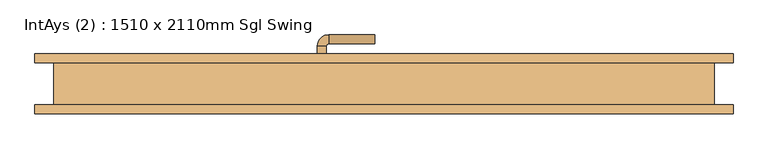
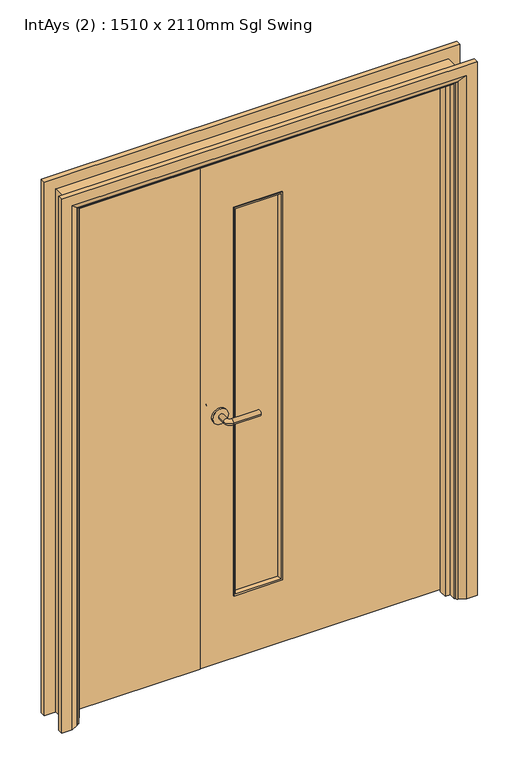
"""IFC4 building model written with IfcOpenShell, lengths in millimetres: door geometry, IntAys (2) : 1510 x 2110mm Sgl Swing."""

import ifcopenshell
import ifcopenshell.guid

model = None  # the IFC model being written
_history = None  # IfcOwnerHistory: only IFC2X3 demands one
_inside = {}  # id of a spatial element -> (the spatial element, [elements in it])
_under = {}  # id of a project, library or spatial element -> (it, [spatial elements below it])
_declared = {}  # id of a project -> (the project, [libraries it declares])
_typed = {}  # id of a type object -> (the type object, [elements of that type])
_made_of = {}  # id of a material, layer set ... -> (it, [elements and type objects made of it])


def new_model(schema):
    """Start an empty IFC model of exactly this schema.

    Asked for "IFC4X3", IfcOpenShell would pick the latest addendum, in which some entities
    have other attributes; the version numbers below select the first issue.
    IFC2X3 requires an IfcOwnerHistory on every rooted entity: one is made here for all.
    """
    global model, _history
    if schema == "IFC4X3":
        model = ifcopenshell.file(schema_version=(4, 3, 0, 0))
    else:
        model = ifcopenshell.file(schema=schema)
    _inside.clear()
    _under.clear()
    _declared.clear()
    _typed.clear()
    _made_of.clear()
    _history = None
    if model.schema == "IFC2X3":
        org = make("IfcOrganization", Name="unknown")
        user = make(
            "IfcPersonAndOrganization",
            ThePerson=make("IfcPerson", FamilyName="unknown"),
            TheOrganization=org,
        )
        app = make(
            "IfcApplication",
            ApplicationDeveloper=org,
            Version="unknown",
            ApplicationFullName="unknown",
            ApplicationIdentifier="unknown",
        )
        _history = make(
            "IfcOwnerHistory",
            OwningUser=user,
            OwningApplication=app,
            ChangeAction="ADDED",
            CreationDate=0,
        )
    return model


def make(cls, **values):
    """One entity of the class cls with the attributes given. An attribute that is None is left unset."""
    return model.create_entity(
        cls, **{name: value for name, value in values.items() if value is not None}
    )


def rooted(cls, **values):
    """An entity with a GlobalId (a new one), such as an element, a storey or a relation."""
    return make(cls, GlobalId=ifcopenshell.guid.new(), OwnerHistory=_history, **values)


def si_unit(unit_type, name, prefix=None):
    """IfcSIUnit, for example si_unit("LENGTHUNIT", "METRE", prefix="MILLI")."""
    return make("IfcSIUnit", UnitType=unit_type, Prefix=prefix, Name=name)


def assignment(units):
    """IfcUnitAssignment: the units of a project."""
    return None if units is None else make("IfcUnitAssignment", Units=units)


def point(xyz):
    """IfcCartesianPoint."""
    return None if xyz is None else make("IfcCartesianPoint", Coordinates=xyz)


def direction(xyz):
    """IfcDirection."""
    return None if xyz is None else make("IfcDirection", DirectionRatios=xyz)


def frame(location, z_axis=None, x_axis=None):
    """IfcAxis2Placement3D, a coordinate frame: its origin and axes. An axis left out is left unset."""
    return make(
        "IfcAxis2Placement3D",
        Location=point(location),
        Axis=direction(z_axis),
        RefDirection=direction(x_axis),
    )


def frame_2d(location, x_axis=None):
    """IfcAxis2Placement2D, a coordinate frame in the plane: its origin and x axis."""
    return make(
        "IfcAxis2Placement2D", Location=point(location), RefDirection=direction(x_axis)
    )


def origin():
    """The frame at (0, 0, 0) with its axes left unset."""
    return frame((0.0, 0.0, 0.0))


def place(relative_to, where):
    """IfcLocalPlacement: puts the frame where relative to a parent placement (None: the world)."""
    return make(
        "IfcLocalPlacement", PlacementRelTo=relative_to, RelativePlacement=where
    )


def context(
    kind, dimensions, precision=None, world=None, true_north=None, identifier=None
):
    """IfcGeometricRepresentationContext, for example the 3D "Model" context."""
    return make(
        "IfcGeometricRepresentationContext",
        ContextIdentifier=identifier,
        ContextType=kind,
        CoordinateSpaceDimension=dimensions,
        Precision=precision,
        WorldCoordinateSystem=world,
        TrueNorth=true_north,
    )


def project(units=None, contexts=None):
    """IfcProject with its units and contexts."""
    return rooted(
        "IfcProject",
        Name="project",
        RepresentationContexts=contexts,
        UnitsInContext=assignment(units),
    )


def spatial(cls, under=None, at=None, **own):
    """A site, building, storey or space (cls), placed at a placement, below another one or the project."""
    s = rooted(cls, ObjectPlacement=at, **own)
    if under is not None:
        _under.setdefault(under.id(), (under, []))[1].append(s)
    return s


def polyline(points):
    """IfcPolyline through the points."""
    return make("IfcPolyline", Points=[point(p) for p in points])


def circle_curve(where, radius):
    """IfcCircle in the frame where."""
    return make("IfcCircle", Position=where, Radius=radius)


def ellipse_curve(where, semi_axis1, semi_axis2):
    """IfcEllipse in the frame where."""
    return make(
        "IfcEllipse", Position=where, SemiAxis1=semi_axis1, SemiAxis2=semi_axis2
    )


def trimmed(basis, trim1, trim2, sense, master):
    """IfcTrimmedCurve: the piece of a basis curve between two trims."""
    return make(
        "IfcTrimmedCurve",
        BasisCurve=basis,
        Trim1=trim1,
        Trim2=trim2,
        SenseAgreement=sense,
        MasterRepresentation=master,
    )


def segment(curve, same_sense, transition):
    """IfcCompositeCurveSegment."""
    return make(
        "IfcCompositeCurveSegment",
        Transition=transition,
        SameSense=same_sense,
        ParentCurve=curve,
    )


def composite_curve(segments, self_intersect=None):
    """IfcCompositeCurve: segments joined end to end."""
    return make("IfcCompositeCurve", Segments=segments, SelfIntersect=self_intersect)


def outline(outer, holes=None, kind="AREA"):
    """IfcArbitraryClosedProfileDef: a profile drawn as a closed curve; with holes, ...WithVoids."""
    if holes is None:
        return make("IfcArbitraryClosedProfileDef", ProfileType=kind, OuterCurve=outer)
    return make(
        "IfcArbitraryProfileDefWithVoids",
        ProfileType=kind,
        OuterCurve=outer,
        InnerCurves=holes,
    )


def extrude(swept, where, along, depth):
    """IfcExtrudedAreaSolid: the profile swept, set in the frame where, extruded along a direction by depth."""
    return make(
        "IfcExtrudedAreaSolid",
        SweptArea=swept,
        Position=where,
        ExtrudedDirection=direction(along),
        Depth=depth,
    )


def faces_of(points, faces, orient=None, outer=None):
    """IfcFace entities. A face is a list of loops; a loop is a list of indices into points, from 0.

    orient and outer hold one flag for each loop. By default every Orientation is true, the
    first loop of a face is its IfcFaceOuterBound and the others are IfcFaceBound.
    """
    made = []
    for i, loops in enumerate(faces):
        bounds = []
        for j, loop in enumerate(loops):
            is_outer = j == 0 if outer is None else outer[i][j]
            bounds.append(
                make(
                    "IfcFaceOuterBound" if is_outer else "IfcFaceBound",
                    Bound=make("IfcPolyLoop", Polygon=[points[k] for k in loop]),
                    Orientation=True if orient is None else orient[i][j],
                )
            )
        made.append(make("IfcFace", Bounds=bounds))
    return made


def faceted_brep(points, faces, orient=None, outer=None, voids=None):
    """IfcFacetedBrep: a solid bounded by flat faces; with voids (closed shells), ...WithVoids."""
    shared = [point(p) for p in points]
    hull = make("IfcClosedShell", CfsFaces=faces_of(shared, faces, orient, outer))
    if voids is None:
        return make("IfcFacetedBrep", Outer=hull)
    return make(
        "IfcFacetedBrepWithVoids",
        Outer=hull,
        Voids=[
            make(cls, CfsFaces=faces_of(shared, fs, o, b)) for cls, fs, o, b in voids
        ],
    )


def shape(context_of_items, identifier, shape_type, items):
    """IfcShapeRepresentation: the items that make up one representation, for example the "Body"."""
    return make(
        "IfcShapeRepresentation",
        ContextOfItems=context_of_items,
        RepresentationIdentifier=identifier,
        RepresentationType=shape_type,
        Items=items,
    )


def source(mapping_origin, context_of_items, identifier, shape_type, items):
    """IfcRepresentationMap: a shape defined once, which mapped items show again and again."""
    return make(
        "IfcRepresentationMap",
        MappingOrigin=mapping_origin,
        MappedRepresentation=shape(context_of_items, identifier, shape_type, items),
    )


def transform(
    local_origin,
    x_axis=None,
    y_axis=None,
    z_axis=None,
    scale=None,
    scale2=None,
    scale3=None,
    uniform=True,
):
    """IfcCartesianTransformationOperator3D, or its non-uniform kind. x_axis, y_axis, z_axis: its Axis1, 2, 3."""
    if uniform:
        return make(
            "IfcCartesianTransformationOperator3D",
            Axis1=direction(x_axis),
            Axis2=direction(y_axis),
            LocalOrigin=point(local_origin),
            Scale=scale,
            Axis3=direction(z_axis),
        )
    return make(
        "IfcCartesianTransformationOperator3DnonUniform",
        Axis1=direction(x_axis),
        Axis2=direction(y_axis),
        LocalOrigin=point(local_origin),
        Scale=scale,
        Axis3=direction(z_axis),
        Scale2=scale2,
        Scale3=scale3,
    )


def mapped(mapping_source, mapping_target):
    """IfcMappedItem: shows the shape of a source again, moved by a transform."""
    return make(
        "IfcMappedItem", MappingSource=mapping_source, MappingTarget=mapping_target
    )


def made_of(thing, what):
    """Note that an element or type object is made of a material, layer set ...; save() writes the relation."""
    if what is not None:
        _made_of.setdefault(what.id(), (what, []))[1].append(thing)
    return thing


def element(
    cls,
    number,
    at=None,
    inside=None,
    cuts=None,
    type_object=None,
    material=None,
    context=None,
    identifier="Body",
    shape_type=None,
    held_by="IfcProductDefinitionShape",
    body=None,
    shapes=None,
    **own,
):
    """One element of the class cls, such as IfcWall. Its Tag is "e" and its number.

    at: its placement. inside: the storey or other place that contains it. cuts: it is an
    opening in that element (IfcRelVoidsElement). A single representation is given by context,
    identifier, shape_type and body (its items); several are given by shapes. held_by: the class
    of the entity that holds the representations. save() writes the other relations.
    """
    e = rooted(cls, Tag="e%d" % number, ObjectPlacement=at, **own)
    if body is not None:
        shapes = [shape(context, identifier, shape_type, body)]
    if shapes is not None:
        e.Representation = make(held_by, Representations=shapes)
    if inside is not None:
        _inside.setdefault(inside.id(), (inside, []))[1].append(e)
    if cuts is not None:
        rooted(
            "IfcRelVoidsElement", RelatingBuildingElement=cuts, RelatedOpeningElement=e
        )
    if type_object is not None:
        _typed.setdefault(type_object.id(), (type_object, []))[1].append(e)
    return made_of(e, material)


def aggregate(whole, parts):
    """IfcRelAggregates: a whole, such as a stair, and the parts it consists of."""
    return rooted("IfcRelAggregates", RelatingObject=whole, RelatedObjects=parts)


def save(model, path):
    """Write the relations noted so far, then the file.

    IfcRelAggregates (storeys below a building ...), IfcRelContainedInSpatialStructure (elements
    in a storey), IfcRelDefinesByType, IfcRelAssociatesMaterial and IfcRelDeclares: one each for
    every whole, place, type object, material and project.
    """
    for whole, parts in _under.values():
        aggregate(whole, parts)
    for where, things in _inside.values():
        rooted(
            "IfcRelContainedInSpatialStructure",
            RelatedElements=things,
            RelatingStructure=where,
        )
    for kind, things in _typed.values():
        rooted("IfcRelDefinesByType", RelatedObjects=things, RelatingType=kind)
    for what, things in _made_of.values():
        rooted("IfcRelAssociatesMaterial", RelatedObjects=things, RelatingMaterial=what)
    for by, libraries in _declared.values():
        rooted("IfcRelDeclares", RelatingContext=by, RelatedDefinitions=libraries)
    model.write(path)


def plane_surface(at):
    """IfcPlane: the flat surface through the origin of the frame at, square to its z axis."""
    return make("IfcPlane", Position=at)


def cylinder_surface(at, radius):
    """IfcCylindricalSurface: all points at the distance radius from the z axis of the frame at."""
    return make("IfcCylindricalSurface", Position=at, Radius=radius)


def revolved_surface(curve, axis_point, axis_direction):
    """IfcSurfaceOfRevolution: the curve turned about the line through axis_point along axis_direction."""
    return make(
        "IfcSurfaceOfRevolution",
        SweptCurve=make("IfcArbitraryOpenProfileDef", ProfileType="CURVE", Curve=curve),
        AxisPosition=make("IfcAxis1Placement", Location=point(axis_point), Axis=direction(axis_direction)),
    )


def advanced_brep(points, edges, surfaces, faces):
    """IfcAdvancedBrep: a solid bounded by faces that lie on surfaces and meet in shared edges.

    An edge is (start, end): straight between two places in points (the first is 0);
    or (start, end, curve); or (start, end, curve, False) where it runs against its curve.
    A face is (place in surfaces, loops), or (place, loops, False) where it looks against
    its surface's normal. A loop lists edges by number (the first is 1), with a minus sign
    where the edge is run from its end to its start. The first loop is the outer one.
    """
    corners = [point(p) for p in points]
    vertices = [make("IfcVertexPoint", VertexGeometry=c) for c in corners]
    made = []
    for start, end, *more in edges:
        made.append(
            make(
                "IfcEdgeCurve",
                EdgeStart=vertices[start],
                EdgeEnd=vertices[end],
                EdgeGeometry=more[0] if more else make("IfcPolyline", Points=[corners[start], corners[end]]),
                SameSense=more[1] if len(more) > 1 else True,
            )
        )
    hull = []
    for where, loops, *sense in faces:
        bounds = []
        for j, loop in enumerate(loops):
            ring = [make("IfcOrientedEdge", EdgeElement=made[abs(k) - 1], Orientation=k > 0) for k in loop]
            bounds.append(
                make(
                    "IfcFaceOuterBound" if j == 0 else "IfcFaceBound",
                    Bound=make("IfcEdgeLoop", EdgeList=ring),
                    Orientation=True,
                )
            )
        hull.append(make("IfcAdvancedFace", Bounds=bounds, FaceSurface=surfaces[where], SameSense=sense[0] if sense else True))
    return make("IfcAdvancedBrep", Outer=make("IfcClosedShell", CfsFaces=hull))


def intays_2_1510_x_2110mm_sgl_swing_f165abe8(model_context):
    return source(origin(), model_context, "Body", "SolidModel", [
        advanced_brep(
        [(88.5, 7.5, 1000.0), (108.5, 7.5, 1000.0), (108.5, -22.5, 1000.0), (88.5, -22.5, 1000.0), (113.5, -27.5, 1000.0), (113.5, -47.5, 1000.0), (218.5, -47.5, 1000.0), (218.5, -27.5, 1000.0)],
        [
            (0, 1, circle_curve(frame((98.5, 7.5, 1000.0), z_axis=(0.0, 1.0, 0.0), x_axis=(1.0, 0.0, 0.0)), 10.0)),
            (1, 0, circle_curve(frame((98.5, 7.5, 1000.0), z_axis=(0.0, 1.0, 0.0), x_axis=(1.0, 0.0, 0.0)), 10.0)),
            (1, 2),
            (2, 3, circle_curve(frame((98.5, -22.5, 1000.0), z_axis=(0.0, 1.0, 0.0), x_axis=(1.0, 0.0, 0.0)), 10.0)),
            (3, 0),
            (3, 2, circle_curve(frame((98.5, -22.5, 1000.0), z_axis=(0.0, 1.0, 0.0), x_axis=(1.0, 0.0, 0.0)), 10.0)),
            (4, 5, circle_curve(frame((113.5, -37.5, 1000.0), z_axis=(-1.0, 0.0, 0.0), x_axis=(0.0, 1.0, 0.0)), 10.0)),
            (5, 3, circle_curve(frame((113.5, -22.5, 1000.0), z_axis=(0.0, 0.0, -1.0), x_axis=(-1.0, 0.0, 0.0)), 25.0)),
            (2, 4, circle_curve(frame((113.5, -22.5, 1000.0), z_axis=(0.0, 0.0, 1.0), x_axis=(-1.0, 0.0, 0.0)), 5.0)),
            (5, 4, circle_curve(frame((113.5, -37.5, 1000.0), z_axis=(-1.0, 0.0, 0.0), x_axis=(0.0, 1.0, 0.0)), 10.0)),
            (6, 7, circle_curve(frame((218.5, -37.5, 1000.0), z_axis=(1.0, 0.0, 0.0), x_axis=(0.0, 1.0, 0.0)), 10.0)),
            (7, 6, circle_curve(frame((218.5, -37.5, 1000.0), z_axis=(1.0, 0.0, 0.0), x_axis=(0.0, 1.0, 0.0)), 10.0)),
            (4, 7),
            (6, 5),
        ],
        [
            plane_surface(frame((98.5, 7.5, 1000.0), z_axis=(0.0, 1.0, 0.0), x_axis=(0.0, 0.0, 1.0))),
            cylinder_surface(frame((98.5, 7.5, 1000.0), z_axis=(0.0, 1.0, 0.0), x_axis=(1.0, 0.0, 0.0)), 10.0),
            revolved_surface(trimmed(ellipse_curve(frame((98.5, -22.5, 1000.0), z_axis=(0.0, -1.0, 0.0), x_axis=(1.0, 0.0, 0.0)), 10.0, 10.0), [point((88.5, -22.5, 1000.0))], [point((108.5, -22.5, 1000.0))], True, "CARTESIAN"), (113.5, -22.5, 1000.0), (0.0, 0.0, -1.0)),
            revolved_surface(trimmed(ellipse_curve(frame((98.5, -22.5, 1000.0), z_axis=(0.0, -1.0, 0.0), x_axis=(1.0, 0.0, 0.0)), 10.0, 10.0), [point((108.5, -22.5, 1000.0))], [point((88.5, -22.5, 1000.0))], True, "CARTESIAN"), (113.5, -22.5, 1000.0), (0.0, 0.0, -1.0)),
            plane_surface(frame((218.5, -37.5, 1000.0), z_axis=(1.0, 0.0, 0.0), x_axis=(0.0, 0.0, 1.0))),
            cylinder_surface(frame((113.5, -37.5, 1000.0), z_axis=(-1.0, 0.0, 0.0), x_axis=(0.0, 1.0, 0.0)), 10.0),
        ],
        [
            (0, [[1, 2]]),
            (1, [[3, 4, 5, -2]]),
            (1, [[-5, 6, -3, -1]]),
            (2, [[7, 8, -4, 9]]),
            (3, [[10, -9, -6, -8]]),
            (4, [[11, 12]]),
            (5, [[13, -11, 14, -7]]),
            (5, [[-14, -12, -13, -10]]),
        ],
    ),
        extrude(outline(composite_curve([segment(trimmed(circle_curve(frame_2d((1000.0, 96.0)), 30.0), [point((1000.0, 66.0))], [point((1000.0, 126.0))], False, "CARTESIAN"), True, "CONTINUOUS"), segment(trimmed(circle_curve(frame_2d((1000.0, 96.0)), 30.0), [point((1000.0, 126.0))], [point((1000.0, 66.0))], False, "CARTESIAN"), True, "CONTINUOUS")], self_intersect=False)), frame((0.0, 7.5, 0.0), z_axis=(0.0, 1.0, 0.0), x_axis=(0.0, 0.0, 1.0)), (0.0, 0.0, 1.0), 8.0),
        advanced_brep(
        [(88.5, 55.5, 1000.0), (108.5, 55.5, 1000.0), (88.5, 85.5, 1000.0), (108.5, 85.5, 1000.0), (113.5, 90.5, 1000.0), (113.5, 110.5, 1000.0), (218.5, 110.5, 1000.0), (218.5, 90.5, 1000.0)],
        [
            (0, 1, circle_curve(frame((98.5, 55.5, 1000.0), z_axis=(0.0, -1.0, 0.0), x_axis=(1.0, 0.0, 0.0)), 10.0)),
            (1, 0, circle_curve(frame((98.5, 55.5, 1000.0), z_axis=(0.0, -1.0, 0.0), x_axis=(1.0, 0.0, 0.0)), 10.0)),
            (0, 2),
            (2, 3, circle_curve(frame((98.5, 85.5, 1000.0), z_axis=(0.0, -1.0, 0.0), x_axis=(1.0, 0.0, 0.0)), 10.0)),
            (3, 1),
            (3, 2, circle_curve(frame((98.5, 85.5, 1000.0), z_axis=(0.0, -1.0, 0.0), x_axis=(1.0, 0.0, 0.0)), 10.0)),
            (4, 3, circle_curve(frame((113.5, 85.5, 1000.0), z_axis=(0.0, 0.0, 1.0), x_axis=(-1.0, 0.0, 0.0)), 5.0)),
            (2, 5, circle_curve(frame((113.5, 85.5, 1000.0), z_axis=(0.0, 0.0, -1.0), x_axis=(-1.0, 0.0, 0.0)), 25.0)),
            (5, 4, circle_curve(frame((113.5, 100.5, 1000.0), z_axis=(-1.0, 0.0, 0.0), x_axis=(0.0, -1.0, 0.0)), 10.0)),
            (4, 5, circle_curve(frame((113.5, 100.5, 1000.0), z_axis=(-1.0, 0.0, 0.0), x_axis=(0.0, -1.0, 0.0)), 10.0)),
            (6, 7, circle_curve(frame((218.5, 100.5, 1000.0), z_axis=(1.0, 0.0, 0.0), x_axis=(0.0, -1.0, 0.0)), 10.0)),
            (7, 6, circle_curve(frame((218.5, 100.5, 1000.0), z_axis=(1.0, 0.0, 0.0), x_axis=(0.0, -1.0, 0.0)), 10.0)),
            (5, 6),
            (7, 4),
        ],
        [
            plane_surface(frame((98.5, 55.5, 1000.0), z_axis=(0.0, -1.0, 0.0), x_axis=(0.0, 0.0, 1.0))),
            cylinder_surface(frame((98.5, 55.5, 1000.0), z_axis=(0.0, -1.0, 0.0), x_axis=(1.0, 0.0, 0.0)), 10.0),
            revolved_surface(trimmed(ellipse_curve(frame((98.5, 85.5, 1000.0), z_axis=(0.0, -1.0, 0.0), x_axis=(1.0, 0.0, 0.0)), 10.0, 10.0), [point((88.5, 85.5, 1000.0))], [point((108.5, 85.5, 1000.0))], True, "CARTESIAN"), (113.5, 85.5, 1000.0), (0.0, 0.0, -1.0)),
            revolved_surface(trimmed(ellipse_curve(frame((98.5, 85.5, 1000.0), z_axis=(0.0, -1.0, 0.0), x_axis=(1.0, 0.0, 0.0)), 10.0, 10.0), [point((108.5, 85.5, 1000.0))], [point((88.5, 85.5, 1000.0))], True, "CARTESIAN"), (113.5, 85.5, 1000.0), (0.0, 0.0, -1.0)),
            plane_surface(frame((218.5, 100.5, 1000.0), z_axis=(1.0, 0.0, 0.0), x_axis=(0.0, 0.0, 1.0))),
            cylinder_surface(frame((113.5, 100.5, 1000.0), z_axis=(-1.0, 0.0, 0.0), x_axis=(0.0, -1.0, 0.0)), 10.0),
        ],
        [
            (0, [[1, 2]]),
            (1, [[-1, 3, 4, 5]]),
            (1, [[-2, -5, 6, -3]]),
            (2, [[7, -4, 8, 9]]),
            (3, [[-8, -6, -7, 10]]),
            (4, [[11, 12]]),
            (5, [[-9, 13, -12, 14]]),
            (5, [[-10, -14, -11, -13]]),
        ],
    ),
        extrude(outline(composite_curve([segment(trimmed(circle_curve(frame_2d((1000.0, 96.0)), 30.0), [point((1000.0, 66.0))], [point((1000.0, 126.0))], False, "CARTESIAN"), True, "CONTINUOUS"), segment(trimmed(circle_curve(frame_2d((1000.0, 96.0)), 30.0), [point((1000.0, 126.0))], [point((1000.0, 66.0))], False, "CARTESIAN"), True, "CONTINUOUS")], self_intersect=False)), frame((0.0, 47.5, 0.0), z_axis=(0.0, 1.0, 0.0), x_axis=(0.0, 0.0, 1.0)), (0.0, 0.0, 1.0), 8.0),
        extrude(outline(polyline([(2102.0, -508.0), (0.0, -508.0), (0.0, -476.0), (2070.0, -476.0), (2070.0, 954.0), (0.0, 954.0), (0.0, 986.0), (2102.0, 986.0), (2102.0, -508.0)])), frame((0.0, -47.5, 0.0), z_axis=(0.0, 1.0, 0.0), x_axis=(0.0, 0.0, 1.0)), (0.0, 0.0, 1.0), 95.0),
        advanced_brep(
        [(-551.0, -67.5, 0.0), (-551.0, -47.5, 0.0), (-481.0, -47.5, 0.0), (-485.0, -53.5, 0.0), (-511.0, -67.5, 0.0), (-551.0, -67.5, 2145.0), (-551.0, -47.5, 2145.0), (1029.0, -47.5, 2145.0), (1029.0, -47.5, 0.0), (959.0, -47.5, 0.0), (959.0, -47.5, 2075.0), (-481.0, -47.5, 2075.0), (-485.0, -53.5, 2079.0), (-511.0, -67.5, 2105.0), (989.0, -67.5, 2105.0), (989.0, -67.5, 0.0), (1029.0, -67.5, 0.0), (1029.0, -67.5, 2145.0), (963.0, -53.5, 0.0), (963.0, -53.5, 2079.0)],
        [
            (0, 1),
            (1, 2),
            (2, 3, circle_curve(frame((-489.0, -46.5, 0.0), z_axis=(0.0, 0.0, -1.0), x_axis=(-1.0, 0.0, 0.0)), 8.0622577)),
            (3, 4),
            (4, 0),
            (0, 5),
            (5, 6),
            (6, 1),
            (6, 7),
            (7, 8),
            (8, 9),
            (9, 10),
            (10, 11),
            (11, 2),
            (11, 12, ellipse_curve(frame((-489.0, -46.5, 2083.0), z_axis=(-0.7071067811865475, 0.0, -0.7071067811865475), x_axis=(0.7071067811865474, 0.0, -0.7071067811865476)), 11.4017543, 8.0622577)),
            (12, 3),
            (12, 13),
            (13, 4),
            (13, 14),
            (14, 15),
            (15, 16),
            (16, 17),
            (17, 5),
            (7, 17),
            (16, 8),
            (15, 18),
            (18, 9, circle_curve(frame((967.0, -46.5, 0.0), z_axis=(0.0, 0.0, -1.0), x_axis=(1.0, 0.0, 0.0)), 8.0622577)),
            (19, 10, ellipse_curve(frame((967.0, -46.5, 2083.0), z_axis=(0.7071067811865475, 0.0, -0.7071067811865475), x_axis=(0.7071067811865474, 0.0, 0.7071067811865476)), 11.4017543, 8.0622577)),
            (18, 19),
            (14, 19),
            (19, 12),
        ],
        [
            plane_surface(frame((-481.0, -47.5, 0.0), z_axis=(0.0, 0.0, -1.0), x_axis=(0.0, -1.0, 0.0))),
            plane_surface(frame((-551.0, -67.5, 0.0), z_axis=(-1.0, 0.0, 0.0), x_axis=(0.0, 0.0, 1.0))),
            plane_surface(frame((-551.0, -47.5, 0.0), z_axis=(0.0, 1.0, 0.0), x_axis=(0.0, 0.0, 1.0))),
            cylinder_surface(frame((-489.0, -46.5, 0.0), z_axis=(0.0, 0.0, -1.0), x_axis=(-1.0, 0.0, 0.0)), 8.0622577),
            plane_surface(frame((-485.0, -53.5, 0.0), z_axis=(0.4740998230350183, -0.8804710999221749, 0.0), x_axis=(0.0, 0.0, 1.0))),
            plane_surface(frame((-511.0, -67.5, 0.0), z_axis=(0.0, -1.0, 0.0), x_axis=(0.0, 0.0, 1.0))),
            plane_surface(frame((1029.0, -67.5, 2145.0), z_axis=(1.0, 0.0, 0.0), x_axis=(0.0, 0.0, -1.0))),
            plane_surface(frame((959.0, -47.5, 0.0), z_axis=(0.0, 0.0, -1.0), x_axis=(0.0, -1.0, 0.0))),
            cylinder_surface(frame((967.0, -46.5, 2075.0), z_axis=(0.0, 0.0, 1.0), x_axis=(1.0, 0.0, 0.0)), 8.0622577),
            plane_surface(frame((963.0, -53.5, 2079.0), z_axis=(-0.4740998230350183, -0.8804710999221749, 0.0), x_axis=(0.0, 0.0, -1.0))),
            plane_surface(frame((-551.0, -67.5, 2145.0), z_axis=(0.0, 0.0, 1.0), x_axis=(1.0, 0.0, 0.0))),
            cylinder_surface(frame((-481.0, -46.5, 2083.0), z_axis=(-1.0, 0.0, 0.0), x_axis=(0.0, 0.0, 1.0)), 8.0622577),
            plane_surface(frame((-485.0, -53.5, 2079.0), z_axis=(0.0, -0.8804710999221749, -0.4740998230350183), x_axis=(1.0, 0.0, 0.0))),
        ],
        [
            (0, [[1, 2, 3, 4, 5]]),
            (1, [[-1, 6, 7, 8]]),
            (2, [[-2, -8, 9, 10, 11, 12, 13, 14]]),
            (3, [[-3, -14, 15, 16]]),
            (4, [[-4, -16, 17, 18]]),
            (5, [[-5, -18, 19, 20, 21, 22, 23, -6]]),
            (6, [[24, -22, 25, -10]]),
            (7, [[-21, 26, 27, -11, -25]]),
            (8, [[28, -12, -27, 29]]),
            (9, [[30, -29, -26, -20]]),
            (10, [[-7, -23, -24, -9]]),
            (11, [[-15, -13, -28, 31]]),
            (12, [[-17, -31, -30, -19]]),
        ],
    ),
        advanced_brep(
        [(1029.0, 67.5, 0.0), (1029.0, 47.5, 0.0), (959.0, 47.5, 0.0), (963.0, 53.5, 0.0), (989.0, 67.5, 0.0), (1029.0, 67.5, 2145.0), (1029.0, 47.5, 2145.0), (-551.0, 47.5, 2145.0), (-551.0, 47.5, 0.0), (-481.0, 47.5, 0.0), (-481.0, 47.5, 2075.0), (959.0, 47.5, 2075.0), (963.0, 53.5, 2079.0), (989.0, 67.5, 2105.0), (-511.0, 67.5, 2105.0), (-511.0, 67.5, 0.0), (-551.0, 67.5, 0.0), (-551.0, 67.5, 2145.0), (-485.0, 53.5, 0.0), (-485.0, 53.5, 2079.0)],
        [
            (0, 1),
            (1, 2),
            (2, 3, circle_curve(frame((967.0, 46.5, 0.0), z_axis=(0.0, 0.0, -1.0), x_axis=(1.0, 0.0, 0.0)), 8.0622577)),
            (3, 4),
            (4, 0),
            (0, 5),
            (5, 6),
            (6, 1),
            (6, 7),
            (7, 8),
            (8, 9),
            (9, 10),
            (10, 11),
            (11, 2),
            (11, 12, ellipse_curve(frame((967.0, 46.5, 2083.0), z_axis=(0.7071067811865475, 0.0, -0.7071067811865475), x_axis=(-0.7071067811865474, 0.0, -0.7071067811865476)), 11.4017543, 8.0622577)),
            (12, 3),
            (12, 13),
            (13, 4),
            (13, 14),
            (14, 15),
            (15, 16),
            (16, 17),
            (17, 5),
            (7, 17),
            (16, 8),
            (15, 18),
            (18, 9, circle_curve(frame((-489.0, 46.5, 0.0), z_axis=(0.0, 0.0, -1.0), x_axis=(-1.0, 0.0, 0.0)), 8.0622577)),
            (19, 10, ellipse_curve(frame((-489.0, 46.5, 2083.0), z_axis=(-0.7071067811865475, 0.0, -0.7071067811865475), x_axis=(-0.7071067811865474, 0.0, 0.7071067811865476)), 11.4017543, 8.0622577)),
            (18, 19),
            (14, 19),
            (19, 12),
        ],
        [
            plane_surface(frame((959.0, 47.5, 0.0), z_axis=(0.0, 0.0, -1.0), x_axis=(0.0, -1.0, 0.0))),
            plane_surface(frame((1029.0, 67.5, 0.0), z_axis=(1.0, 0.0, 0.0), x_axis=(0.0, 0.0, 1.0))),
            plane_surface(frame((1029.0, 47.5, 0.0), z_axis=(0.0, -1.0, 0.0), x_axis=(0.0, 0.0, 1.0))),
            cylinder_surface(frame((967.0, 46.5, 0.0), z_axis=(0.0, 0.0, -1.0), x_axis=(1.0, 0.0, 0.0)), 8.0622577),
            plane_surface(frame((963.0, 53.5, 0.0), z_axis=(-0.4740998230350126, 0.8804710999221779, 0.0), x_axis=(0.0, 0.0, 1.0))),
            plane_surface(frame((989.0, 67.5, 0.0), z_axis=(0.0, 1.0, 0.0), x_axis=(0.0, 0.0, 1.0))),
            plane_surface(frame((-551.0, 67.5, 2145.0), z_axis=(-1.0, 0.0, 0.0), x_axis=(0.0, 0.0, -1.0))),
            plane_surface(frame((-481.0, 47.5, 0.0), z_axis=(0.0, 0.0, -1.0), x_axis=(0.0, -1.0, 0.0))),
            cylinder_surface(frame((-489.0, 46.5, 2075.0), z_axis=(0.0, 0.0, 1.0), x_axis=(-1.0, 0.0, 0.0)), 8.0622577),
            plane_surface(frame((-485.0, 53.5, 2079.0), z_axis=(0.4740998230350183, 0.8804710999221749, 0.0), x_axis=(0.0, 0.0, -1.0))),
            plane_surface(frame((1029.0, 67.5, 2145.0), z_axis=(0.0, 0.0, 1.0), x_axis=(-1.0, 0.0, 0.0))),
            cylinder_surface(frame((959.0, 46.5, 2083.0), z_axis=(1.0, 0.0, 0.0), x_axis=(0.0, 0.0, 1.0)), 8.0622577),
            plane_surface(frame((963.0, 53.5, 2079.0), z_axis=(0.0, 0.8804710999221763, -0.4740998230350154), x_axis=(-1.0, 0.0, 0.0))),
        ],
        [
            (0, [[1, 2, 3, 4, 5]]),
            (1, [[-1, 6, 7, 8]]),
            (2, [[-2, -8, 9, 10, 11, 12, 13, 14]]),
            (3, [[-3, -14, 15, 16]]),
            (4, [[-4, -16, 17, 18]]),
            (5, [[-5, -18, 19, 20, 21, 22, 23, -6]]),
            (6, [[24, -22, 25, -10]]),
            (7, [[-21, 26, 27, -11, -25]]),
            (8, [[28, -12, -27, 29]]),
            (9, [[30, -29, -26, -20]]),
            (10, [[-7, -23, -24, -9]]),
            (11, [[-15, -13, -28, 31]]),
            (12, [[-17, -31, -30, -19]]),
        ],
    ),
        faceted_brep([(-457.0, 12.5, 0.0), (-457.0, -19.5, 0.0), (-476.0, -19.5, 0.0), (-476.0, 12.5, 0.0), (-457.0, 12.5, 2051.0), (-457.0, -19.5, 2051.0), (-476.0, -19.5, 2070.0), (-476.0, 12.5, 2070.0), (935.0, 12.5, 0.0), (954.0, 12.5, 0.0), (954.0, -19.5, 0.0), (935.0, -19.5, 0.0), (935.0, 12.5, 2051.0), (954.0, 12.5, 2070.0), (954.0, -19.5, 2070.0), (935.0, -19.5, 2051.0)], [[[0, 1, 2, 3]], [[1, 0, 4, 5]], [[2, 1, 5, 6]], [[3, 2, 6, 7]], [[0, 3, 7, 4]], [[8, 9, 10, 11]], [[12, 13, 9, 8]], [[13, 14, 10, 9]], [[14, 15, 11, 10]], [[15, 12, 8, 11]], [[5, 4, 12, 15]], [[6, 5, 15, 14]], [[7, 6, 14, 13]], [[4, 7, 13, 12]]]),
        extrude(outline(polyline([(335.0, 25.5), (150.0, 25.5), (150.0, 37.5), (335.0, 37.5), (335.0, 25.5)])), frame((0.0, 0.0, 257.0), z_axis=(0.0, 0.0, 1.0), x_axis=(1.0, 0.0, 0.0)), (0.0, 0.0, 1.0), 1560.0),
        extrude(outline(polyline([(22.0, 15.5), (-473.0, 15.5), (-473.0, 47.5), (22.0, 47.5), (22.0, 15.5)])), frame((0.0, 0.0, 5.753223), z_axis=(0.0, 0.0, 1.0), x_axis=(1.0, 0.0, 0.0)), (0.0, 0.0, 1.0), 2061.246777),
        extrude(outline(polyline([(5.753223, 951.0), (2067.0, 951.0), (2067.0, 25.0), (5.753223, 25.0), (5.753223, 951.0)]), holes=[polyline([(1817.0, 150.0), (1817.0, 335.0), (257.0, 335.0), (257.0, 150.0), (1817.0, 150.0)])]), frame((0.0, 15.5, 0.0), z_axis=(0.0, 1.0, 0.0), x_axis=(0.0, 0.0, 1.0)), (0.0, 0.0, 1.0), 32.0),
        faceted_brep([(335.0, 12.5, 257.0), (335.0, 25.5, 257.0), (335.0, 25.5, 1817.0), (335.0, 12.5, 1817.0), (323.0, 25.5, 269.0), (329.0, 12.5, 263.0), (329.0, 12.5, 1811.0), (323.0, 25.5, 1805.0), (150.0, 25.5, 1817.0), (150.0, 12.5, 1817.0), (156.0, 12.5, 1811.0), (162.0, 25.5, 1805.0), (150.0, 25.5, 257.0), (150.0, 12.5, 257.0), (156.0, 12.5, 263.0), (162.0, 25.5, 269.0)], [[[0, 1, 2, 3]], [[4, 5, 6, 7]], [[3, 2, 8, 9]], [[7, 6, 10, 11]], [[9, 8, 12, 13]], [[11, 10, 14, 15]], [[1, 12, 8, 2], [7, 11, 15, 4]], [[13, 12, 1, 0]], [[3, 9, 13, 0], [5, 14, 10, 6]], [[15, 14, 5, 4]]]),
        faceted_brep([(150.0, 50.5, 257.0), (150.0, 37.5, 257.0), (150.0, 37.5, 1817.0), (150.0, 50.5, 1817.0), (162.0, 37.5, 269.0), (156.0, 50.5, 263.0), (156.0, 50.5, 1811.0), (162.0, 37.5, 1805.0), (335.0, 37.5, 1817.0), (335.0, 50.5, 1817.0), (329.0, 50.5, 1811.0), (323.0, 37.5, 1805.0), (335.0, 37.5, 257.0), (335.0, 50.5, 257.0), (329.0, 50.5, 263.0), (323.0, 37.5, 269.0)], [[[0, 1, 2, 3]], [[4, 5, 6, 7]], [[3, 2, 8, 9]], [[7, 6, 10, 11]], [[9, 8, 12, 13]], [[11, 10, 14, 15]], [[1, 12, 8, 2], [7, 11, 15, 4]], [[13, 12, 1, 0]], [[3, 9, 13, 0], [5, 14, 10, 6]], [[15, 14, 5, 4]]]),
    ])


if __name__ == "__main__":
    model = new_model("IFC4")
    model_context = context("Model", 3, world=origin())
    ifc_project = project(units=[si_unit("LENGTHUNIT", "METRE", prefix="MILLI")], contexts=[model_context])
    site = spatial("IfcSite", under=ifc_project)
    building = spatial("IfcBuilding", under=site)
    placement = place(None, origin())
    intays_2_1510_x_2110mm_sgl_swing_shape = intays_2_1510_x_2110mm_sgl_swing_f165abe8(model_context)
    element("IfcDoor", 1, ObjectType="IntAys (2) : 1510 x 2110mm Sgl Swing", at=placement, inside=building, context=model_context, shape_type="MappedRepresentation", body=[
        mapped(intays_2_1510_x_2110mm_sgl_swing_shape, transform((0.0, 0.0, 0.0), x_axis=(1.0, 0.0, 0.0), y_axis=(0.0, 1.0, 0.0), z_axis=(0.0, 0.0, 1.0))),
    ])
    save(model, "model.ifc")

# Revit data of these elements
# Type "IntAys (2) : 1510 x 2110mm Sgl Swing"
#   Type Mark = "46"
#   Type Comments = "Internal Asymmetric"
#   Operation = "DoubleDoorSingleSwing"
#   Construction Type Id = "SGL"
#   Keynote = "L20"
#   Description = "Internal Asymmetric Door"
#   Analytic Construction = "Large single-glazed windows"
#   Visual Light Transmittance = 0.9
#   VisionPanel Width = 185 mm
#   Thickness = 32 mm
#   Stop Thickness = 19 mm
#   Stop Depth = 32 mm
#   Stile Top Rail = 250 mm
#   Stile Shutting = 125 mm
#   Stile Bottom Rail = 250 mm
#   Solar Heat Gain Coefficient = 0.86
#   Secondary Panel Width = 495 mm
#   Rough Width = 1510 mm
#   Rough Height = 2110 mm
#   Main Panel Width = 926 mm
#   Heat Transfer Coefficient (U) = 5.5617 W/(m²·K)
#   Handle Z Distance = 1000 mm
#   Handle X Distance = 75 mm
#   Handle Length = 350 mm
#   Frame Thickness = 32 mm
#   Door Panel Width = 926 mm
#   Door Panel Thickness = 32 mm
#   Height = 2110 mm
#   Door Panel Offset = 0 mm
#   Structural Tolerance = 8 mm
#   Tolerance = 3 mm
#   UnderCut = 7 mm
#   Width = 1510 mm
#   Door Panel Height = 2060 mm
#   Architrave Setback = 5 mm
#   Vis - Swing Single = yes
#   Vis - Swing Opposing = no
#   Vis - Swing Double = no
#   Vis - Stops = yes
#   Vis - Ironmongery = yes
#   Define Thermal Properties by = 1
#   Material Ironmongery = Door - Handle
#   Material Glass = Door - Glazing
#   Material Frame = Door - Frame/Mullion
#   Material Door = Door - Panel
#   Material Beading = Door - Panel
#   Material Architrave = Door - Architrave
#   Handle Style = element 261135
#   Function = (empty or 0)
#   Wall Closure = (empty or 0)
# Element 1 (IfcDoor, "IntAys (2) : 1510 x 2110mm Sgl Swing")
#   Materials on its faces: "Door - Panel", "Door - Architrave", "Door - Handle", "Door - Frame/Mullion", "Door - Glazing"
# Materials
#   "Door - Handle": class "Miscellaneous", colour RGB 0 0 0, transparency 0, Keynote = "P21"
#   "Door - Glazing": class "Miscellaneous", colour RGB 0 0 255, transparency 0.75
#   "Door - Frame/Mullion": class "Wood", colour RGB 212 179 113, transparency 0, Keynote = "L20"
#   "Door - Panel": class "Wood", colour RGB 210 159 95, transparency 0, Keynote = "L20"
#   "Door - Architrave": class "Wood", colour RGB 154 90 5, transparency 0, Keynote = "P20"
